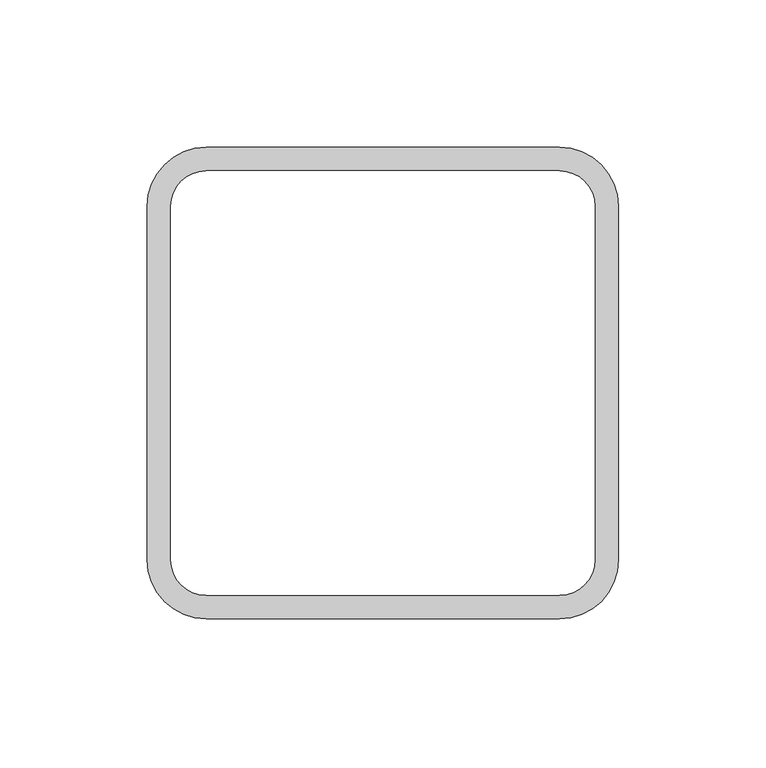
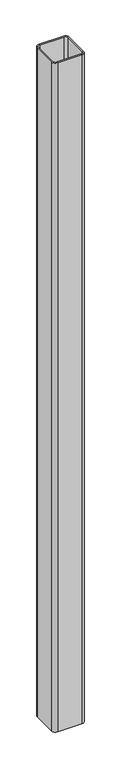
"""IFC4 building model written with IfcOpenShell, lengths in millimetres: column geometry, NLRS_28_SCO_TLB_stalen kolom buisprofiel koudgevormd vierkant-BCPG-MMBS-SRP_gen_rsf : stalen kolom buisprofiel koudgevormd vierkant RHSC_gen__160x160x8."""

from ifc_helpers import new_model, si_unit, point, frame, frame_2d, origin, place, context, project, spatial, polyline, circle_curve, trimmed, segment, composite_curve, outline, extrude, source, transform, mapped, element, save


def column_9cc0dcb1(model_context):
    return source(origin(), model_context, "Body", "SweptSolid", [
        extrude(outline(composite_curve([segment(trimmed(circle_curve(frame_2d((60.0, 60.0)), 20.0), [point((60.0, 80.0))], [point((80.0, 60.0))], False, "CARTESIAN"), True, "CONTINUOUS"), segment(polyline([(80.0, 60.0), (80.0, -60.0)]), True, "CONTINUOUS"), segment(trimmed(circle_curve(frame_2d((60.0, -60.0)), 20.0), [point((80.0, -60.0))], [point((60.0, -80.0))], False, "CARTESIAN"), True, "CONTINUOUS"), segment(polyline([(60.0, -80.0), (-60.0, -80.0)]), True, "CONTINUOUS"), segment(trimmed(circle_curve(frame_2d((-60.0, -60.0)), 20.0), [point((-60.0, -80.0))], [point((-80.0, -60.0))], False, "CARTESIAN"), True, "CONTINUOUS"), segment(polyline([(-80.0, -60.0), (-80.0, 60.0)]), True, "CONTINUOUS"), segment(trimmed(circle_curve(frame_2d((-60.0, 60.0)), 20.0), [point((-80.0, 60.0))], [point((-60.0, 80.0))], False, "CARTESIAN"), True, "CONTINUOUS"), segment(polyline([(-60.0, 80.0), (60.0, 80.0)]), True, "CONTINUOUS")], self_intersect=False), holes=[composite_curve([segment(polyline([(60.0, 72.0), (-60.0, 72.0)]), True, "CONTINUOUS"), segment(trimmed(circle_curve(frame_2d((-60.0, 60.0)), 12.0), [point((-60.0, 72.0))], [point((-72.0, 60.0))], True, "CARTESIAN"), True, "CONTINUOUS"), segment(polyline([(-72.0, 60.0), (-72.0, -60.0)]), True, "CONTINUOUS"), segment(trimmed(circle_curve(frame_2d((-60.0, -60.0)), 12.0), [point((-72.0, -60.0))], [point((-60.0, -72.0))], True, "CARTESIAN"), True, "CONTINUOUS"), segment(polyline([(-60.0, -72.0), (60.0, -72.0)]), True, "CONTINUOUS"), segment(trimmed(circle_curve(frame_2d((60.0, -60.0)), 12.0), [point((60.0, -72.0))], [point((72.0, -60.0))], True, "CARTESIAN"), True, "CONTINUOUS"), segment(polyline([(72.0, -60.0), (72.0, 60.0)]), True, "CONTINUOUS"), segment(trimmed(circle_curve(frame_2d((60.0, 60.0)), 12.0), [point((72.0, 60.0))], [point((60.0, 72.0))], True, "CARTESIAN"), True, "CONTINUOUS")], self_intersect=False)]), frame((0.0, 0.0, 3760.0), z_axis=(0.0, 0.0, 1.0), x_axis=(1.0, 0.0, 0.0)), (0.0, 0.0, 1.0), 3510.0),
    ])


if __name__ == "__main__":
    model = new_model("IFC4")
    model_context = context("Model", 3, world=origin())
    ifc_project = project(units=[si_unit("LENGTHUNIT", "METRE", prefix="MILLI")], contexts=[model_context])
    site = spatial("IfcSite", under=ifc_project)
    building = spatial("IfcBuilding", under=site)
    placement = place(None, origin())
    column_shape = column_9cc0dcb1(model_context)
    element("IfcColumn", 1, ObjectType="NLRS_28_SCO_TLB_stalen kolom buisprofiel koudgevormd vierkant-BCPG-MMBS-SRP_gen_rsf : stalen kolom buisprofiel koudgevormd vierkant RHSC_gen__160x160x8", at=placement, inside=building, context=model_context, shape_type="MappedRepresentation", body=[
        mapped(column_shape, transform((0.0, 0.0, 0.0), x_axis=(1.0, 0.0, 0.0), y_axis=(0.0, 1.0, 0.0), z_axis=(0.0, 0.0, 1.0))),
    ])
    save(model, "model.ifc")

# Revit data of these elements
# Type "NLRS_28_SCO_TLB_stalen kolom buisprofiel koudgevormd vierkant-BCPG-MMBS-SRP_gen_rsf : stalen kolom buisprofiel koudgevormd vierkant RHSC_gen__160x160x8"
#   Type IFC Predefined Type = "COLUMN"
#   Export Type to IFC As = "IfcColumnType"
#   Type IfcGUID = "2$hNzCXOT3YR8V$0Cfyzxk"
#   Type Comments = "K160x160x8"
#   Model = " "
#   Manufacturer = " "
#   Description = "stalen kolom K160x160x8"
#   Assembly Code = "28.11"
#   vz = 80 mm
#   vy = 80 mm
#   vpz = 80 mm
#   vpy = 80 mm
#   tw = 8 mm
#   tf = 8 mm
#   ri = 20 mm
#   ra = 12 mm
#   d = 160 mm
#   bf = 160 mm
#   NLRS_C_lengte [instance default] = 2743.2 mm
#   Structural Material = NLRS_h2_staal_gen_rsf
#   Keynote = ""
# Element 1 (IfcColumn, "NLRS_28_SCO_TLB_stalen kolom buisprofiel koudgevormd vierkant-BCPG-MMBS-SRP_gen_rsf : stalen kolom buisprofiel koudgevormd vierkant RHSC_gen__160x160x8")
#   NLRS_C_lengte = 3510 mm
#   Materials on its faces: "NLRS_h2_staal_gen_rsf"
# Materials
#   "NLRS_h2_staal_gen_rsf": class "H - Metaal", colour RGB 189 187 185, transparency 0, Keynote = "h2", Manufacturer = "Revit Standards Foundation", URL = "www.revitstandards.org", Description = "staal", Cost = 0
